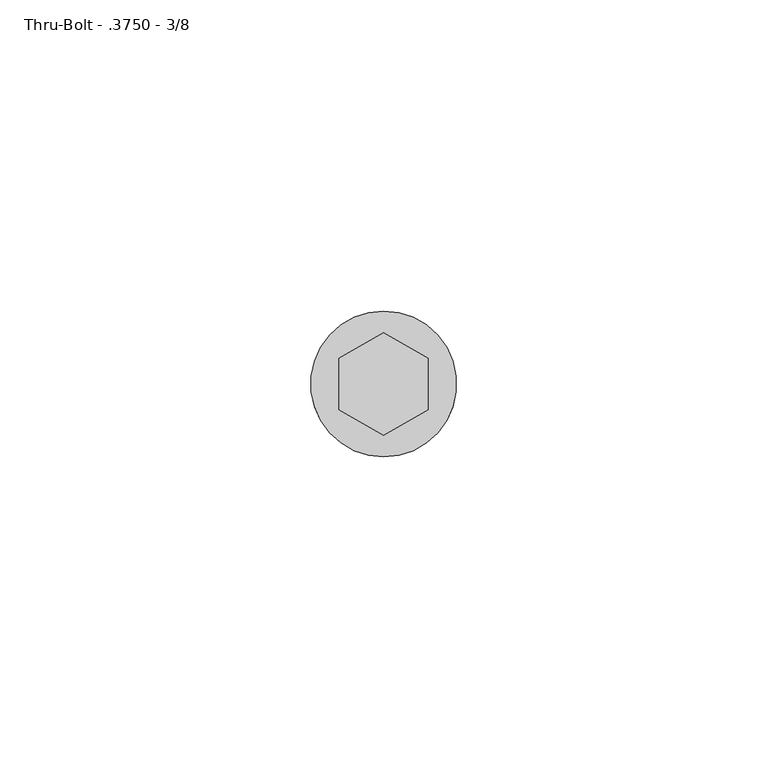
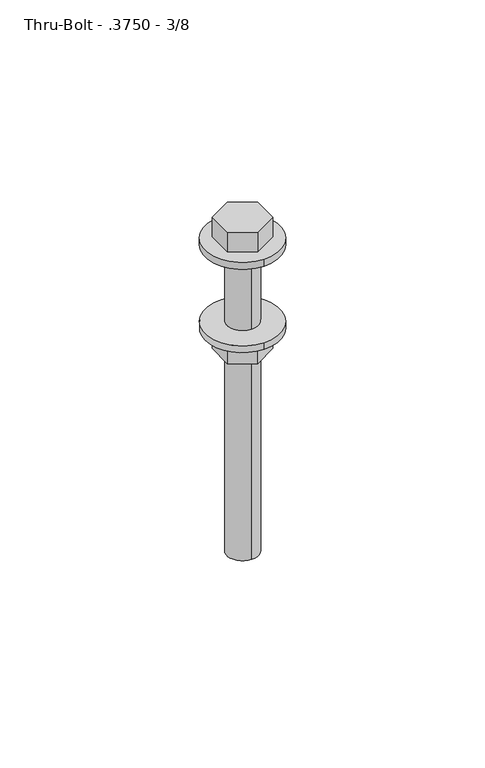
"""IFC4 building model written with IfcOpenShell, lengths in millimetres: fastener geometry, 060523 - W_P_C - Fastenings - Generic : Thru-Bolt - .3750 - 3/8."""

from ifc_helpers import new_model, si_unit, point, frame, origin, origin_with_axes, origin_2d, place, context, project, spatial, polyline, circle_curve, trimmed, segment, composite_curve, outline, extrude, source, transform, mapped, element, save


def thru_bolt_3750_3_8_96d0f578(model_context):
    return source(origin(), model_context, "Body", "SweptSolid", [
        extrude(outline(composite_curve([segment(trimmed(circle_curve(origin_2d(), 11.7185281), [point((0.0, 11.7185281))], [point((0.0, -11.7185281))], False, "CARTESIAN"), True, "CONTINUOUS"), segment(trimmed(circle_curve(origin_2d(), 11.7185281), [point((0.0, -11.7185281))], [point((0.0, 11.7185281))], False, "CARTESIAN"), True, "CONTINUOUS")], self_intersect=False)), origin_with_axes(), (0.0, 0.0, 1.0), 2.2690667),
        extrude(outline(composite_curve([segment(trimmed(circle_curve(origin_2d(), 11.7185281), [point((0.0, 11.7185281))], [point((0.0, -11.7185281))], False, "CARTESIAN"), True, "CONTINUOUS"), segment(trimmed(circle_curve(origin_2d(), 11.7185281), [point((0.0, -11.7185281))], [point((0.0, 11.7185281))], False, "CARTESIAN"), True, "CONTINUOUS")], self_intersect=False)), frame((0.0, 0.0, -27.6690667), z_axis=(0.0, 0.0, 1.0), x_axis=(1.0, 0.0, 0.0)), (0.0, 0.0, 1.0), 2.2690667),
        extrude(outline(polyline([(-7.14375, -4.124446), (-7.14375, 4.124446), (0.0, 8.248892), (7.14375, 4.124446), (7.14375, -4.124446), (0.0, -8.248892), (-7.14375, -4.124446)])), frame((0.0, 0.0, -34.4762667), z_axis=(0.0, 0.0, 1.0), x_axis=(1.0, 0.0, 0.0)), (0.0, 0.0, 1.0), 6.8072),
        extrude(outline(polyline([(-7.14375, 4.124446), (0.0, 8.248892), (7.14375, 4.124446), (7.14375, -4.124446), (0.0, -8.248892), (-7.14375, -4.124446), (-7.14375, 4.124446)])), frame((0.0, 0.0, 2.2690667), z_axis=(0.0, 0.0, 1.0), x_axis=(1.0, 0.0, 0.0)), (0.0, 0.0, 1.0), 6.8072),
        extrude(outline(composite_curve([segment(trimmed(circle_curve(origin_2d(), 4.9113281), [point((0.0, -4.9113281))], [point((0.0, 4.9113281))], False, "CARTESIAN"), True, "CONTINUOUS"), segment(trimmed(circle_curve(origin_2d(), 4.9113281), [point((0.0, 4.9113281))], [point((0.0, -4.9113281))], False, "CARTESIAN"), True, "CONTINUOUS")], self_intersect=False)), frame((0.0, 0.0, -101.6), z_axis=(0.0, 0.0, 1.0), x_axis=(1.0, 0.0, 0.0)), (0.0, 0.0, 1.0), 103.8690667),
    ])


if __name__ == "__main__":
    model = new_model("IFC4")
    model_context = context("Model", 3, world=origin())
    ifc_project = project(units=[si_unit("LENGTHUNIT", "METRE", prefix="MILLI")], contexts=[model_context])
    site = spatial("IfcSite", under=ifc_project)
    building = spatial("IfcBuilding", under=site)
    placement = place(None, origin())
    thru_bolt_3750_3_8_shape = thru_bolt_3750_3_8_96d0f578(model_context)
    element("IfcFastener", 1, ObjectType="060523 - W_P_C - Fastenings - Generic : Thru-Bolt - .3750 - 3/8", at=placement, inside=building, context=model_context, shape_type="MappedRepresentation", body=[
        mapped(thru_bolt_3750_3_8_shape, transform((0.0, 0.0, 0.0), x_axis=(1.0, 0.0, 0.0), y_axis=(0.0, 1.0, 0.0), z_axis=(0.0, 0.0, 1.0))),
    ])
    save(model, "model.ifc")

# Revit data of these elements
# Type "060523 - W_P_C - Fastenings - Generic : Thru-Bolt - .3750 - 3/8"
#   Washer_Thickness = 0' - 0.08933"
#   Washer Radius = 0' - 0.46136"
#   Washer Offset - Head = 0' - 0.08933"
#   Washer Offset = 0' - 0.08933"
#   Thickness_of_Substrate [instance default] = 0' - 1"
#   Side = 0' - 0.3252"
#   Radius = 0' - 0.19336"
#   Length [instance default] = 0' - 4"
#   Head Size = 0' - 0 9/16"
#   Head Radius = 0' - 0 9/32"
#   Head Height = 0' - 0.268"
#   Double Diameter = 0' - 0 99/128"
#   Diameter = 0' - 0 99/256"
#   Default Elevation = 4' - 0"
#   Washer_Nut_Visibility = yes
#   Washer_Head_Visibility = yes
#   Round_Head_Visibility = no
#   Point Visibility = no
#   Nut_Visibility = yes
#   Hex_Head_Visiblilty = yes
#   Washer Material = none
#   Bolt Material (Size) = AT SILL - FASTENER AT 24" O.C.
# Element 1 (IfcFastener, "060523 - W_P_C - Fastenings - Generic : Thru-Bolt - .3750 - 3/8")
#   Materials on its faces: "AT SILL - FASTENER AT 24\" O.C."
# Materials
#   "AT SILL - FASTENER AT 24\" O.C.": class "Generic", colour RGB 120 120 120, transparency 0, Cost = 0
